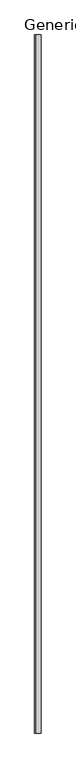
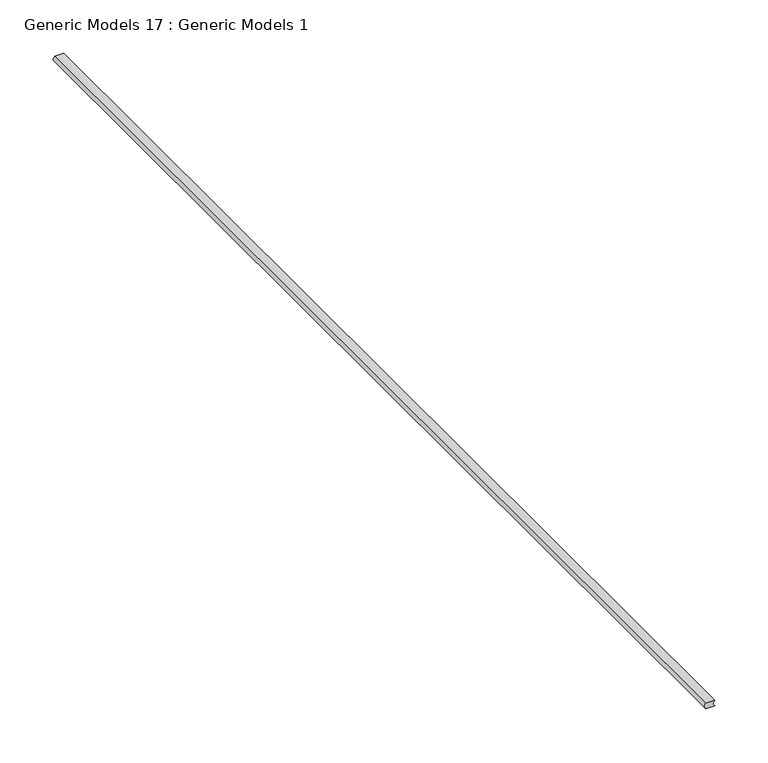
"""IFC4 building model written with IfcOpenShell, lengths in millimetres: proxy geometry, Generic Models 17 : Generic Models 1."""

from ifc_helpers import new_model, si_unit, point, frame, frame_2d, origin, place, context, project, spatial, polyline, circle_curve, trimmed, segment, composite_curve, outline, extrude, source, transform, mapped, element, save


def generic_models_17_generic_models_1_5a74d62d(model_context):
    return source(origin(), model_context, "Body", "SweptSolid", [
        extrude(outline(composite_curve([segment(trimmed(circle_curve(frame_2d((3.175, 49802.7897405)), 4.3100275), [point((0.0, 49799.875))], [point((6.35, 49799.875))], True, "CARTESIAN"), True, "CONTINUOUS"), segment(polyline([(6.35, 49799.875), (6.35, 49790.35)]), True, "CONTINUOUS"), segment(trimmed(circle_curve(frame_2d((3.175, 49793.2647405)), 4.3100275), [point((6.35, 49790.35))], [point((0.0, 49790.35))], False, "CARTESIAN"), True, "CONTINUOUS"), segment(polyline([(0.0, 49790.35), (0.0, 49799.875)]), True, "CONTINUOUS")], self_intersect=False)), frame((0.0, 0.0, 0.0), z_axis=(0.0, 1.0, 0.0), x_axis=(0.0, 0.0, 1.0)), (0.0, 0.0, 1.0), 1219.2),
    ])


if __name__ == "__main__":
    model = new_model("IFC4")
    model_context = context("Model", 3, world=origin())
    ifc_project = project(units=[si_unit("LENGTHUNIT", "METRE", prefix="MILLI")], contexts=[model_context])
    site = spatial("IfcSite", under=ifc_project)
    building = spatial("IfcBuilding", under=site)
    placement = place(None, origin())
    generic_models_17_generic_models_1_shape = generic_models_17_generic_models_1_5a74d62d(model_context)
    element("IfcBuildingElementProxy", 1, Name="Generic Models 17 : Generic Models 1", ObjectType="Generic Models 17 : Generic Models 1", at=placement, inside=building, context=model_context, shape_type="MappedRepresentation", body=[
        mapped(generic_models_17_generic_models_1_shape, transform((0.0, 0.0, 0.0), x_axis=(1.0, 0.0, 0.0), y_axis=(0.0, 1.0, 0.0), z_axis=(0.0, 0.0, 1.0))),
    ])
    save(model, "model.ifc")

# Revit data of these elements
# Element 1 (IfcBuildingElementProxy, "Generic Models 17 : Generic Models 1")
#   Materials on its faces: "ACOUSTICAL SEALANT"
# Materials
#   "ACOUSTICAL SEALANT": class "Unassigned", colour RGB 120 120 120, transparency 0, Cost = 0
